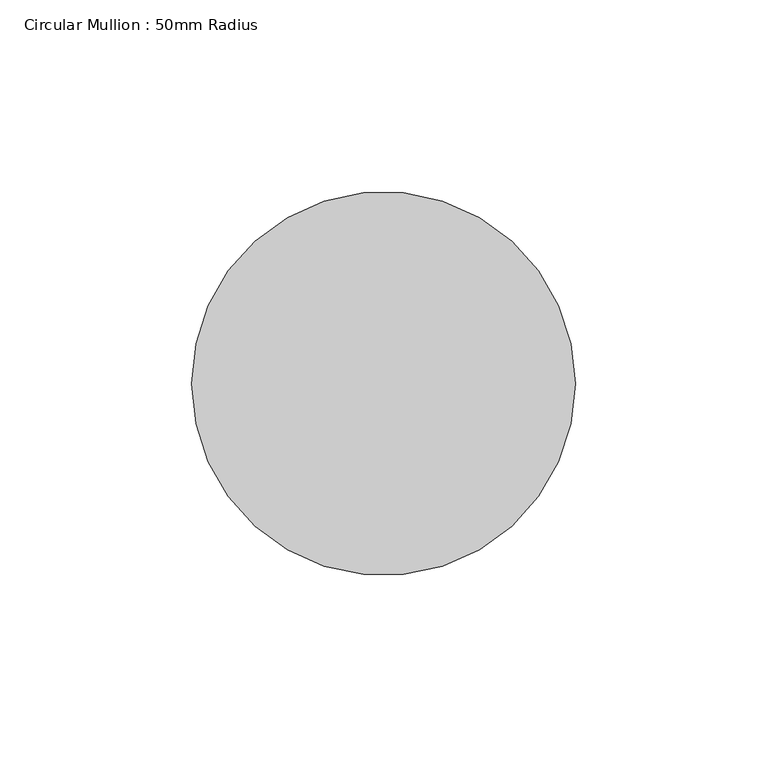
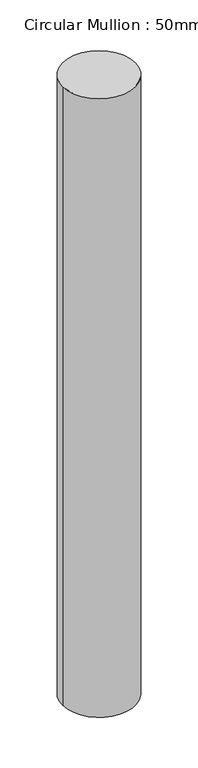
"""IFC4 building model written with IfcOpenShell, lengths in millimetres: member geometry, Circular Mullion : 50mm Radius."""

from ifc_helpers import new_model, si_unit, point, frame, origin, origin_2d, place, context, project, spatial, circle_curve, trimmed, segment, composite_curve, outline, extrude, source, transform, mapped, element, save


def circular_mullion_50mm_radius_8d576fdb(model_context):
    return source(origin(), model_context, "Body", "SweptSolid", [
        extrude(outline(composite_curve([segment(trimmed(circle_curve(origin_2d(), 50.0), [point((50.0, 0.0))], [point((-50.0, 0.0))], False, "CARTESIAN"), True, "CONTINUOUS"), segment(trimmed(circle_curve(origin_2d(), 50.0), [point((-50.0, 0.0))], [point((50.0, 0.0))], False, "CARTESIAN"), True, "CONTINUOUS")], self_intersect=False)), frame((0.0, 0.0, -903.0305402), z_axis=(0.0, 0.0, 1.0), x_axis=(1.0, 0.0, 0.0)), (0.0, 0.0, 1.0), 903.0305402),
    ])


if __name__ == "__main__":
    model = new_model("IFC4")
    model_context = context("Model", 3, world=origin())
    ifc_project = project(units=[si_unit("LENGTHUNIT", "METRE", prefix="MILLI")], contexts=[model_context])
    site = spatial("IfcSite", under=ifc_project)
    building = spatial("IfcBuilding", under=site)
    placement = place(None, origin())
    circular_mullion_50mm_radius_shape = circular_mullion_50mm_radius_8d576fdb(model_context)
    element("IfcMember", 1, ObjectType="Circular Mullion : 50mm Radius", at=placement, inside=building, context=model_context, shape_type="MappedRepresentation", body=[
        mapped(circular_mullion_50mm_radius_shape, transform((0.0, 0.0, 0.0), x_axis=(1.0, 0.0, 0.0), y_axis=(0.0, 1.0, 0.0), z_axis=(0.0, 0.0, 1.0))),
    ])
    save(model, "model.ifc")

# Revit data of these elements
# Type "Circular Mullion : 50mm Radius"
#   built-in parameter 1007350 = 0.164042 (stored number, unit not read)
# Element 1 (IfcMember, "Circular Mullion : 50mm Radius")
#   Materials on its faces: "Aluminium"
# Materials
#   "Aluminium": class "Metal", colour RGB 247 247 247, transparency 0, Description = "Aluminium 6061", Cost = 0
